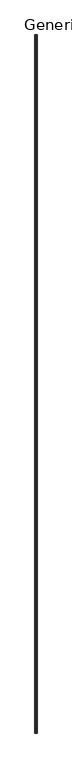
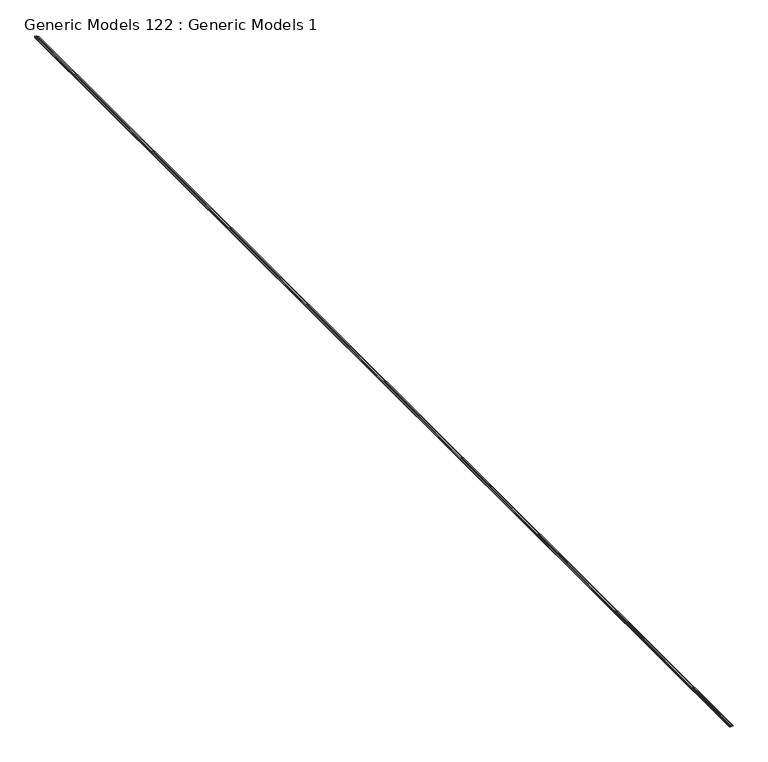
"""IFC4 building model written with IfcOpenShell, lengths in millimetres: proxy geometry, Generic Models 122 : Generic Models 1."""

from ifc_helpers import new_model, si_unit, origin, place, context, project, spatial, faceted_brep, source, transform, mapped, element, save


def generic_models_122_generic_models_1_2220e7a8(model_context):
    return source(origin(), model_context, "Body", "Brep", [
        faceted_brep([(-6986.3995748, 11981.8769662, 142599.5579199), (-6966.7145748, 11981.8769662, 142599.5579199), (-6966.7145748, 11981.8769662, 142610.9879199), (-6951.4745748, 11981.8769662, 142610.9879199), (-6951.4745748, 11981.8769662, 142599.5579199), (-6929.0313908, 11981.8769662, 142599.5579199), (-6929.0313908, 11981.8769662, 142598.2879199), (-6952.7445748, 11981.8769662, 142598.2879199), (-6952.7445748, 11981.8769662, 142609.7179199), (-6965.4445748, 11981.8769662, 142609.7179199), (-6965.4445748, 11981.8769662, 142598.2879199), (-6987.6695748, 11981.8769662, 142598.2879199), (-6987.6695748, 11981.8769662, 142603.0377199), (-6986.8107339, 11981.8769662, 142603.0377199), (-6986.8107339, 11981.8769662, 142622.0822986), (-6985.5407339, 11981.8769662, 142622.0822986), (-6985.5407339, 11981.8769662, 142601.7677199), (-6986.3995748, 11981.8769662, 142601.7677199), (-6986.3995748, -7068.1230338, 142599.5579199), (-6986.3995748, -7068.1230338, 142601.7677199), (-6985.5407339, -7068.1230338, 142601.7677199), (-6985.5407339, -7068.1230338, 142622.0822986), (-6986.8107339, -7068.1230338, 142622.0822986), (-6986.8107339, -7068.1230338, 142603.0377199), (-6987.6695748, -7068.1230338, 142603.0377199), (-6987.6695748, -7068.1230338, 142598.2879199), (-6965.4445748, -7068.1230338, 142598.2879199), (-6965.4445748, -7068.1230338, 142609.7179199), (-6952.7445748, -7068.1230338, 142609.7179199), (-6952.7445748, -7068.1230338, 142598.2879199), (-6929.0313908, -7068.1230338, 142598.2879199), (-6929.0313908, -7068.1230338, 142599.5579199), (-6951.4745748, -7068.1230338, 142599.5579199), (-6951.4745748, -7068.1230338, 142610.9879199), (-6966.7145748, -7068.1230338, 142610.9879199), (-6966.7145748, -7068.1230338, 142599.5579199), (-6986.3995748, 11778.6769662, 142601.7677199), (-6986.3995748, -464.1230338, 142601.7677199), (-6986.3995748, -464.1230338, 142599.5579199), (-6986.3995748, 11778.6769662, 142599.5579199), (-6985.5407339, 11778.6769662, 142601.7677199), (-6985.5407339, -464.1230338, 142601.7677199), (-6985.5407339, 11778.6769662, 142622.0822986), (-6985.5407339, -464.1230338, 142622.0822986), (-6986.8107339, 11778.6769662, 142622.0822986), (-6986.8107339, -464.1230338, 142622.0822986), (-6986.8107339, 11778.6769662, 142603.0377199), (-6986.8107339, -464.1230338, 142603.0377199), (-6987.6695748, 11778.6769662, 142603.0377199), (-6987.6695748, -464.1230338, 142603.0377199)], [[[0, 1, 2, 3, 4, 5, 6, 7, 8, 9, 10, 11, 12, 13, 14, 15, 16, 17]], [[18, 19, 20, 21, 22, 23, 24, 25, 26, 27, 28, 29, 30, 31, 32, 33, 34, 35]], [[0, 17, 36, 37, 19, 18, 38, 39]], [[17, 16, 40, 41, 20, 19, 37, 36]], [[16, 15, 42, 43, 21, 20, 41, 40]], [[15, 14, 44, 45, 22, 21, 43, 42]], [[14, 13, 46, 47, 23, 22, 45, 44]], [[13, 12, 48, 49, 24, 23, 47, 46]], [[12, 11, 25, 24, 49, 48]], [[11, 10, 26, 25]], [[10, 9, 27, 26]], [[9, 8, 28, 27]], [[8, 7, 29, 28]], [[7, 6, 30, 29]], [[6, 5, 31, 30]], [[5, 4, 32, 31]], [[4, 3, 33, 32]], [[3, 2, 34, 33]], [[2, 1, 35, 34]], [[1, 0, 39, 38, 18, 35]]]),
    ])


if __name__ == "__main__":
    model = new_model("IFC4")
    model_context = context("Model", 3, world=origin())
    ifc_project = project(units=[si_unit("LENGTHUNIT", "METRE", prefix="MILLI")], contexts=[model_context])
    site = spatial("IfcSite", under=ifc_project)
    building = spatial("IfcBuilding", under=site)
    placement = place(None, origin())
    generic_models_122_generic_models_1_shape = generic_models_122_generic_models_1_2220e7a8(model_context)
    element("IfcBuildingElementProxy", 1, Name="Generic Models 122 : Generic Models 1", ObjectType="Generic Models 122 : Generic Models 1", at=placement, inside=building, context=model_context, shape_type="MappedRepresentation", body=[
        mapped(generic_models_122_generic_models_1_shape, transform((0.0, 0.0, 0.0), x_axis=(1.0, 0.0, 0.0), y_axis=(0.0, 1.0, 0.0), z_axis=(0.0, 0.0, 1.0))),
    ])
    save(model, "model.ifc")

# Revit data of these elements
# Element 1 (IfcBuildingElementProxy, "Generic Models 122 : Generic Models 1")
#   Materials on its faces: "_16 GA. COPPER SOFFIT DRIP SCREED"
# Materials
#   "_16 GA. COPPER SOFFIT DRIP SCREED": class "Generic", colour RGB 253 192 103, transparency 0, Cost = 0
